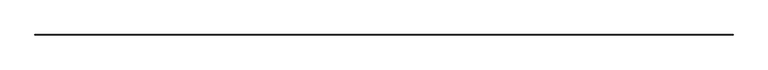
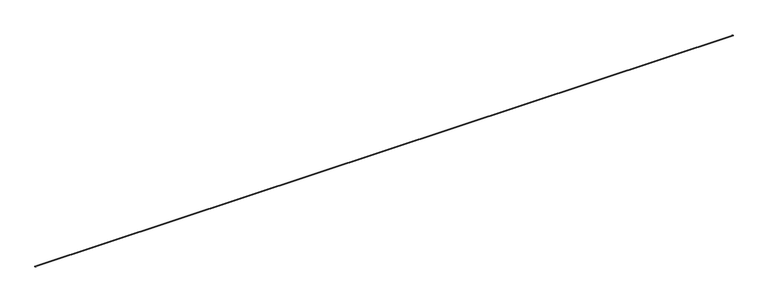
"""IFC4 building model written with IfcOpenShell, lengths in millimetres: proxy geometry, Fakeline : Fakeline."""

from ifc_helpers import new_model, si_unit, point, frame, origin, origin_2d, place, context, project, spatial, circle_curve, trimmed, segment, composite_curve, outline, extrude, source, transform, mapped, element, save


def generic_models_3d06f719(model_context):
    return source(origin(), model_context, "Body", "SweptSolid", [
        extrude(outline(composite_curve([segment(trimmed(circle_curve(origin_2d(), 3.175), [point((-3.175, 0.0))], [point((3.175, 0.0))], False, "CARTESIAN"), True, "CONTINUOUS"), segment(trimmed(circle_curve(origin_2d(), 3.175), [point((3.175, 0.0))], [point((-3.175, 0.0))], False, "CARTESIAN"), True, "CONTINUOUS")], self_intersect=False)), frame((0.0, 0.0, 0.0), z_axis=(1.0, 0.0, 0.0), x_axis=(0.0, 1.0, 0.0)), (0.0, 0.0, 1.0), 8382.0),
    ])


if __name__ == "__main__":
    model = new_model("IFC4")
    model_context = context("Model", 3, world=origin())
    ifc_project = project(units=[si_unit("LENGTHUNIT", "METRE", prefix="MILLI")], contexts=[model_context])
    site = spatial("IfcSite", under=ifc_project)
    building = spatial("IfcBuilding", under=site)
    placement = place(None, origin())
    generic_models_shape = generic_models_3d06f719(model_context)
    element("IfcBuildingElementProxy", 1, Name="Fakeline : Fakeline", ObjectType="Fakeline : Fakeline", at=placement, inside=building, context=model_context, shape_type="MappedRepresentation", body=[
        mapped(generic_models_shape, transform((0.0, 0.0, 0.0), x_axis=(1.0, 0.0, 0.0), y_axis=(0.0, 1.0, 0.0), z_axis=(0.0, 0.0, 1.0))),
    ])
    save(model, "model.ifc")

# Revit data of these elements
# Project information
#   Project Issue Date = "Issue Date"
#   Project Status = "Project Status"
#   Client Name = "Owner"
#   Project Address = "Enter address here"
#   Project Name = "Project Name"
#   Project Number = "Project Number"
# Type "Fakeline : Fakeline"
#   Grid [instance default] = "A"
#   Text Size = 5' - 0"
#   built-in parameter 1001306 [instance default] = 50 (stored number, unit not read)
#   Default Elevation = 4' - 0"
#   Assembly Code = ""
# Element 1 (IfcBuildingElementProxy, "Fakeline : Fakeline")
#   built-in parameter 1001306 = 27.5 (stored number, unit not read)
#   Materials on its faces: "Grid"
# Materials
#   "Grid": class "Unassigned", colour RGB 255 128 0, transparency 0, Comments = "Rendering appearance not upgraded "
